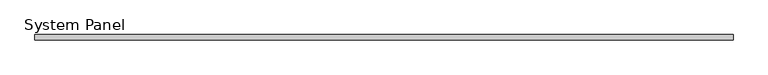
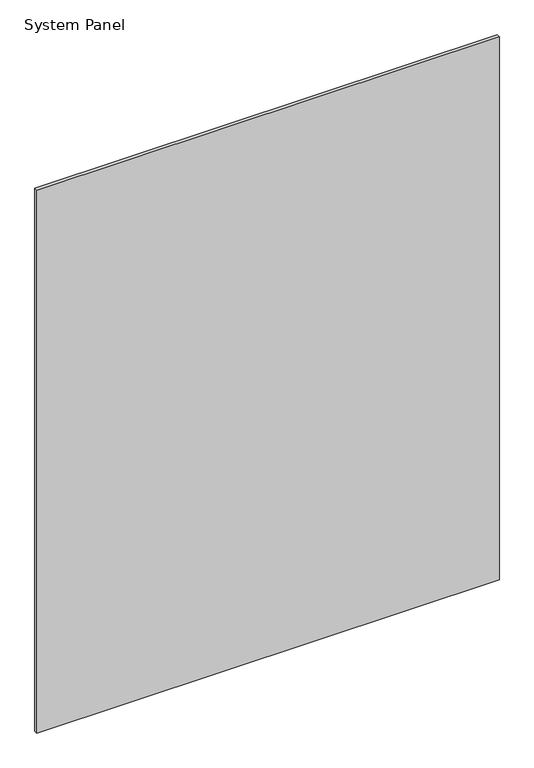
"""IFC4 building model written with IfcOpenShell, lengths in millimetres: plate geometry, System Panel : WWm-Glass-20mm-10mmOffset."""

from ifc_helpers import new_model, si_unit, origin, origin_with_axes, place, context, project, spatial, polyline, outline, extrude, source, transform, mapped, element, save


def system_panel_23211be6(model_context):
    return source(origin(), model_context, "Body", "SweptSolid", [
        extrude(outline(polyline([(1350.0, 0.0), (-1350.0, 0.0), (-1350.0, 20.0), (1350.0, 20.0), (1350.0, 0.0)])), origin_with_axes(), (0.0, 0.0, 1.0), 3350.0),
    ])


if __name__ == "__main__":
    model = new_model("IFC4")
    model_context = context("Model", 3, world=origin())
    ifc_project = project(units=[si_unit("LENGTHUNIT", "METRE", prefix="MILLI")], contexts=[model_context])
    site = spatial("IfcSite", under=ifc_project)
    building = spatial("IfcBuilding", under=site)
    placement = place(None, origin())
    system_panel_shape = system_panel_23211be6(model_context)
    element("IfcPlate", 1, ObjectType="System Panel : WWm-Glass-20mm-10mmOffset", at=placement, inside=building, context=model_context, shape_type="MappedRepresentation", body=[
        mapped(system_panel_shape, transform((0.0, 0.0, 0.0), x_axis=(1.0, 0.0, 0.0), y_axis=(0.0, 1.0, 0.0), z_axis=(0.0, 0.0, 1.0))),
    ])
    save(model, "model.ifc")

# Revit data of these elements
# Type "System Panel : WWm-Glass-20mm-10mmOffset"
#   Finish = ""
# Element 1 (IfcPlate, "System Panel : WWm-Glass-20mm-10mmOffset")
#   Materials on its faces: "WW-EC-GL-Storefront"
# Materials
#   "WW-EC-GL-Storefront": class "Glass", colour RGB 236 240 239, transparency 0.85, Description = "Storefront Glass", Cost = 0
